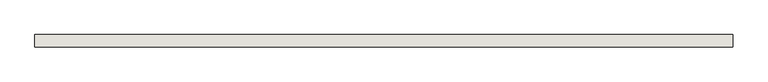
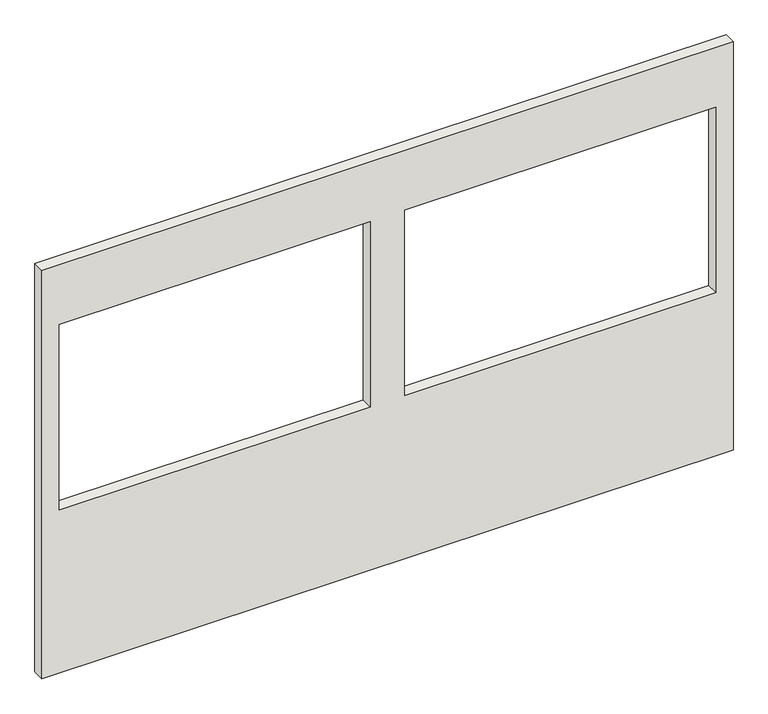
"""IFC4 building model written with IfcOpenShell, lengths in millimetres: wall geometry, 0_3d."""

from ifc_helpers import new_model, si_unit, frame, origin, place, context, project, spatial, polyline, outline, extrude, source, transform, mapped, element, save


def wall_957d8b85(model_context):
    return source(origin(), model_context, "Body", "SweptSolid", [
        extrude(outline(polyline([(0.0, 0.0), (0.0, 4000.0), (2500.0, 4000.0), (2500.0, 0.0), (0.0, 0.0)]), holes=[polyline([(2135.0, 1900.0), (1000.0, 1900.0), (1000.0, 100.0), (2135.0, 100.0), (2135.0, 1900.0)]), polyline([(2135.0, 3900.0), (1000.0, 3900.0), (1000.0, 2100.0), (2135.0, 2100.0), (2135.0, 3900.0)])]), frame((0.0, 0.0, 0.0), z_axis=(0.0, 1.0, 0.0), x_axis=(0.0, 0.0, 1.0)), (0.0, 0.0, 1.0), 70.0),
    ])


if __name__ == "__main__":
    model = new_model("IFC4")
    model_context = context("Model", 3, world=origin())
    ifc_project = project(units=[si_unit("LENGTHUNIT", "METRE", prefix="MILLI")], contexts=[model_context])
    site = spatial("IfcSite", under=ifc_project)
    building = spatial("IfcBuilding", under=site)
    placement = place(None, origin())
    wall_shape = wall_957d8b85(model_context)
    element("IfcWall", 1, ObjectType="0_3d", at=placement, inside=building, context=model_context, shape_type="MappedRepresentation", body=[
        mapped(wall_shape, transform((0.0, 0.0, 0.0), x_axis=(1.0, 0.0, 0.0), y_axis=(0.0, 1.0, 0.0), z_axis=(0.0, 0.0, 1.0))),
    ])
    save(model, "model.ifc")

# Revit data of these elements
# Element 1 (IfcWall, "0_3d")
#   Materials on its faces: "Glass_Simple"
# Materials
#   "Glass_Simple": class "Unassigned", colour RGB 255 255 255, transparency 0.9
